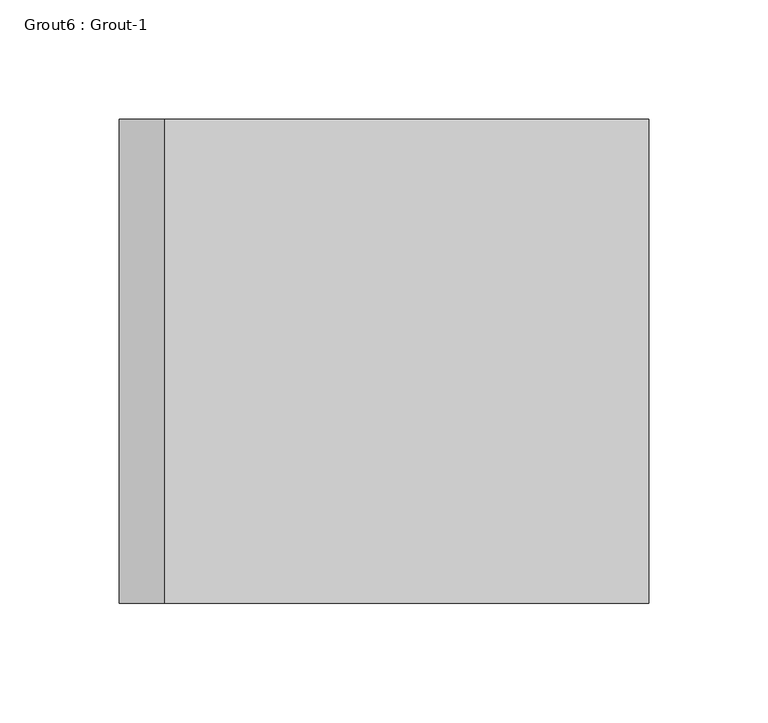
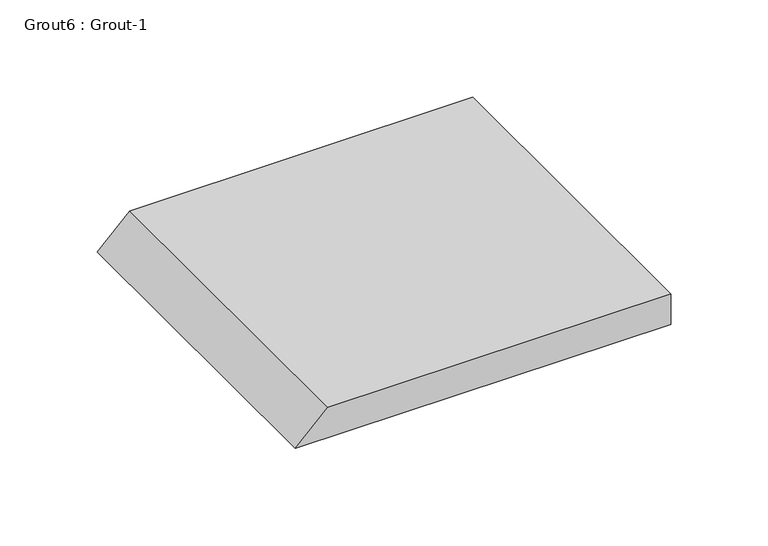
"""IFC4 building model written with IfcOpenShell, lengths in millimetres: proxy geometry, Grout6 : Grout-1."""

import ifcopenshell
import ifcopenshell.guid

model = None  # the IFC model being written
_history = None  # IfcOwnerHistory: only IFC2X3 demands one
_inside = {}  # id of a spatial element -> (the spatial element, [elements in it])
_under = {}  # id of a project, library or spatial element -> (it, [spatial elements below it])
_declared = {}  # id of a project -> (the project, [libraries it declares])
_typed = {}  # id of a type object -> (the type object, [elements of that type])
_made_of = {}  # id of a material, layer set ... -> (it, [elements and type objects made of it])


def new_model(schema):
    """Start an empty IFC model of exactly this schema.

    Asked for "IFC4X3", IfcOpenShell would pick the latest addendum, in which some entities
    have other attributes; the version numbers below select the first issue.
    IFC2X3 requires an IfcOwnerHistory on every rooted entity: one is made here for all.
    """
    global model, _history
    if schema == "IFC4X3":
        model = ifcopenshell.file(schema_version=(4, 3, 0, 0))
    else:
        model = ifcopenshell.file(schema=schema)
    _inside.clear()
    _under.clear()
    _declared.clear()
    _typed.clear()
    _made_of.clear()
    _history = None
    if model.schema == "IFC2X3":
        org = make("IfcOrganization", Name="unknown")
        user = make(
            "IfcPersonAndOrganization",
            ThePerson=make("IfcPerson", FamilyName="unknown"),
            TheOrganization=org,
        )
        app = make(
            "IfcApplication",
            ApplicationDeveloper=org,
            Version="unknown",
            ApplicationFullName="unknown",
            ApplicationIdentifier="unknown",
        )
        _history = make(
            "IfcOwnerHistory",
            OwningUser=user,
            OwningApplication=app,
            ChangeAction="ADDED",
            CreationDate=0,
        )
    return model


def make(cls, **values):
    """One entity of the class cls with the attributes given. An attribute that is None is left unset."""
    return model.create_entity(
        cls, **{name: value for name, value in values.items() if value is not None}
    )


def rooted(cls, **values):
    """An entity with a GlobalId (a new one), such as an element, a storey or a relation."""
    return make(cls, GlobalId=ifcopenshell.guid.new(), OwnerHistory=_history, **values)


def si_unit(unit_type, name, prefix=None):
    """IfcSIUnit, for example si_unit("LENGTHUNIT", "METRE", prefix="MILLI")."""
    return make("IfcSIUnit", UnitType=unit_type, Prefix=prefix, Name=name)


def assignment(units):
    """IfcUnitAssignment: the units of a project."""
    return None if units is None else make("IfcUnitAssignment", Units=units)


def point(xyz):
    """IfcCartesianPoint."""
    return None if xyz is None else make("IfcCartesianPoint", Coordinates=xyz)


def direction(xyz):
    """IfcDirection."""
    return None if xyz is None else make("IfcDirection", DirectionRatios=xyz)


def frame(location, z_axis=None, x_axis=None):
    """IfcAxis2Placement3D, a coordinate frame: its origin and axes. An axis left out is left unset."""
    return make(
        "IfcAxis2Placement3D",
        Location=point(location),
        Axis=direction(z_axis),
        RefDirection=direction(x_axis),
    )


def origin():
    """The frame at (0, 0, 0) with its axes left unset."""
    return frame((0.0, 0.0, 0.0))


def place(relative_to, where):
    """IfcLocalPlacement: puts the frame where relative to a parent placement (None: the world)."""
    return make(
        "IfcLocalPlacement", PlacementRelTo=relative_to, RelativePlacement=where
    )


def context(
    kind, dimensions, precision=None, world=None, true_north=None, identifier=None
):
    """IfcGeometricRepresentationContext, for example the 3D "Model" context."""
    return make(
        "IfcGeometricRepresentationContext",
        ContextIdentifier=identifier,
        ContextType=kind,
        CoordinateSpaceDimension=dimensions,
        Precision=precision,
        WorldCoordinateSystem=world,
        TrueNorth=true_north,
    )


def project(units=None, contexts=None):
    """IfcProject with its units and contexts."""
    return rooted(
        "IfcProject",
        Name="project",
        RepresentationContexts=contexts,
        UnitsInContext=assignment(units),
    )


def spatial(cls, under=None, at=None, **own):
    """A site, building, storey or space (cls), placed at a placement, below another one or the project."""
    s = rooted(cls, ObjectPlacement=at, **own)
    if under is not None:
        _under.setdefault(under.id(), (under, []))[1].append(s)
    return s


def polyline(points):
    """IfcPolyline through the points."""
    return make("IfcPolyline", Points=[point(p) for p in points])


def outline(outer, holes=None, kind="AREA"):
    """IfcArbitraryClosedProfileDef: a profile drawn as a closed curve; with holes, ...WithVoids."""
    if holes is None:
        return make("IfcArbitraryClosedProfileDef", ProfileType=kind, OuterCurve=outer)
    return make(
        "IfcArbitraryProfileDefWithVoids",
        ProfileType=kind,
        OuterCurve=outer,
        InnerCurves=holes,
    )


def extrude(swept, where, along, depth):
    """IfcExtrudedAreaSolid: the profile swept, set in the frame where, extruded along a direction by depth."""
    return make(
        "IfcExtrudedAreaSolid",
        SweptArea=swept,
        Position=where,
        ExtrudedDirection=direction(along),
        Depth=depth,
    )


def shape(context_of_items, identifier, shape_type, items):
    """IfcShapeRepresentation: the items that make up one representation, for example the "Body"."""
    return make(
        "IfcShapeRepresentation",
        ContextOfItems=context_of_items,
        RepresentationIdentifier=identifier,
        RepresentationType=shape_type,
        Items=items,
    )


def source(mapping_origin, context_of_items, identifier, shape_type, items):
    """IfcRepresentationMap: a shape defined once, which mapped items show again and again."""
    return make(
        "IfcRepresentationMap",
        MappingOrigin=mapping_origin,
        MappedRepresentation=shape(context_of_items, identifier, shape_type, items),
    )


def transform(
    local_origin,
    x_axis=None,
    y_axis=None,
    z_axis=None,
    scale=None,
    scale2=None,
    scale3=None,
    uniform=True,
):
    """IfcCartesianTransformationOperator3D, or its non-uniform kind. x_axis, y_axis, z_axis: its Axis1, 2, 3."""
    if uniform:
        return make(
            "IfcCartesianTransformationOperator3D",
            Axis1=direction(x_axis),
            Axis2=direction(y_axis),
            LocalOrigin=point(local_origin),
            Scale=scale,
            Axis3=direction(z_axis),
        )
    return make(
        "IfcCartesianTransformationOperator3DnonUniform",
        Axis1=direction(x_axis),
        Axis2=direction(y_axis),
        LocalOrigin=point(local_origin),
        Scale=scale,
        Axis3=direction(z_axis),
        Scale2=scale2,
        Scale3=scale3,
    )


def mapped(mapping_source, mapping_target):
    """IfcMappedItem: shows the shape of a source again, moved by a transform."""
    return make(
        "IfcMappedItem", MappingSource=mapping_source, MappingTarget=mapping_target
    )


def made_of(thing, what):
    """Note that an element or type object is made of a material, layer set ...; save() writes the relation."""
    if what is not None:
        _made_of.setdefault(what.id(), (what, []))[1].append(thing)
    return thing


def element(
    cls,
    number,
    at=None,
    inside=None,
    cuts=None,
    type_object=None,
    material=None,
    context=None,
    identifier="Body",
    shape_type=None,
    held_by="IfcProductDefinitionShape",
    body=None,
    shapes=None,
    **own,
):
    """One element of the class cls, such as IfcWall. Its Tag is "e" and its number.

    at: its placement. inside: the storey or other place that contains it. cuts: it is an
    opening in that element (IfcRelVoidsElement). A single representation is given by context,
    identifier, shape_type and body (its items); several are given by shapes. held_by: the class
    of the entity that holds the representations. save() writes the other relations.
    """
    e = rooted(cls, Tag="e%d" % number, ObjectPlacement=at, **own)
    if body is not None:
        shapes = [shape(context, identifier, shape_type, body)]
    if shapes is not None:
        e.Representation = make(held_by, Representations=shapes)
    if inside is not None:
        _inside.setdefault(inside.id(), (inside, []))[1].append(e)
    if cuts is not None:
        rooted(
            "IfcRelVoidsElement", RelatingBuildingElement=cuts, RelatedOpeningElement=e
        )
    if type_object is not None:
        _typed.setdefault(type_object.id(), (type_object, []))[1].append(e)
    return made_of(e, material)


def aggregate(whole, parts):
    """IfcRelAggregates: a whole, such as a stair, and the parts it consists of."""
    return rooted("IfcRelAggregates", RelatingObject=whole, RelatedObjects=parts)


def save(model, path):
    """Write the relations noted so far, then the file.

    IfcRelAggregates (storeys below a building ...), IfcRelContainedInSpatialStructure (elements
    in a storey), IfcRelDefinesByType, IfcRelAssociatesMaterial and IfcRelDeclares: one each for
    every whole, place, type object, material and project.
    """
    for whole, parts in _under.values():
        aggregate(whole, parts)
    for where, things in _inside.values():
        rooted(
            "IfcRelContainedInSpatialStructure",
            RelatedElements=things,
            RelatingStructure=where,
        )
    for kind, things in _typed.values():
        rooted("IfcRelDefinesByType", RelatedObjects=things, RelatingType=kind)
    for what, things in _made_of.values():
        rooted("IfcRelAssociatesMaterial", RelatedObjects=things, RelatingMaterial=what)
    for by, libraries in _declared.values():
        rooted("IfcRelDeclares", RelatingContext=by, RelatedDefinitions=libraries)
    model.write(path)


def grout6_grout_1_0f871906(model_context):
    return source(origin(), model_context, "Body", "SweptSolid", [
        extrude(outline(polyline([(19.05, 590115.4434739), (0.0, 590096.3934739), (0.0, 590318.6434739), (19.05, 590318.6434739), (19.05, 590115.4434739)])), frame((0.0, -535306.3413841, 0.0), z_axis=(0.0, 1.0, 0.0), x_axis=(0.0, 0.0, 1.0)), (0.0, 0.0, 1.0), 203.2),
    ])


if __name__ == "__main__":
    model = new_model("IFC4")
    model_context = context("Model", 3, world=origin())
    ifc_project = project(units=[si_unit("LENGTHUNIT", "METRE", prefix="MILLI")], contexts=[model_context])
    site = spatial("IfcSite", under=ifc_project)
    building = spatial("IfcBuilding", under=site)
    placement = place(None, origin())
    grout6_grout_1_shape = grout6_grout_1_0f871906(model_context)
    element("IfcBuildingElementProxy", 1, Name="Grout6 : Grout-1", ObjectType="Grout6 : Grout-1", at=placement, inside=building, context=model_context, shape_type="MappedRepresentation", body=[
        mapped(grout6_grout_1_shape, transform((0.0, 0.0, 0.0), x_axis=(1.0, 0.0, 0.0), y_axis=(0.0, 1.0, 0.0), z_axis=(0.0, 0.0, 1.0))),
    ])
    save(model, "model.ifc")

# Revit data of these elements
# Element 1 (IfcBuildingElementProxy, "Grout6 : Grout-1")
#   Materials on its faces: "3/4\" NON SHRINK GROUT"
# Materials
#   "3/4\" NON SHRINK GROUT": class "Generic", colour RGB 145 145 143, transparency 0, Cost = 0
